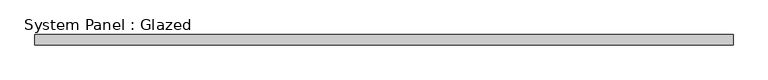
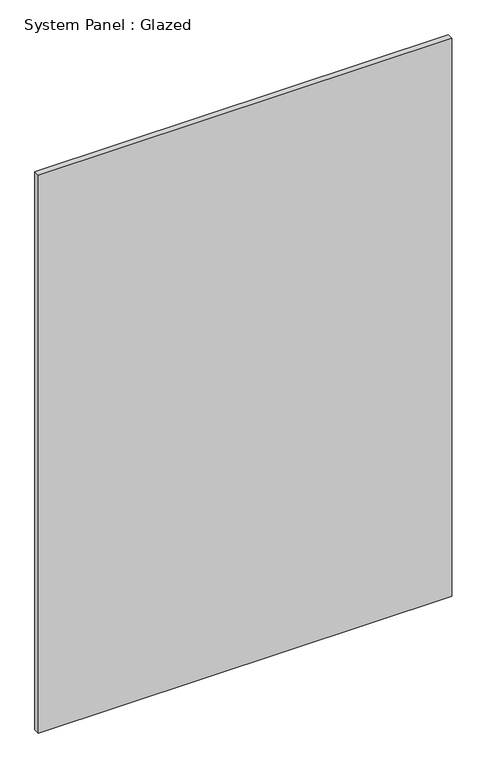
"""IFC4 building model written with IfcOpenShell, lengths in millimetres: plate geometry, System Panel : Glazed."""

from ifc_helpers import new_model, si_unit, origin, origin_with_axes, place, context, project, spatial, polyline, outline, extrude, source, transform, mapped, element, save


def system_panel_glazed_5990fd4e(model_context):
    return source(origin(), model_context, "Body", "SweptSolid", [
        extrude(outline(polyline([(832.5, 24.5), (-832.5, 24.5), (-832.5, 49.5), (832.5, 49.5), (832.5, 24.5)])), origin_with_axes(), (0.0, 0.0, 1.0), 2375.0),
    ])


if __name__ == "__main__":
    model = new_model("IFC4")
    model_context = context("Model", 3, world=origin())
    ifc_project = project(units=[si_unit("LENGTHUNIT", "METRE", prefix="MILLI")], contexts=[model_context])
    site = spatial("IfcSite", under=ifc_project)
    building = spatial("IfcBuilding", under=site)
    placement = place(None, origin())
    system_panel_glazed_shape = system_panel_glazed_5990fd4e(model_context)
    element("IfcPlate", 1, ObjectType="System Panel : Glazed", at=placement, inside=building, context=model_context, shape_type="MappedRepresentation", body=[
        mapped(system_panel_glazed_shape, transform((0.0, 0.0, 0.0), x_axis=(1.0, 0.0, 0.0), y_axis=(0.0, 1.0, 0.0), z_axis=(0.0, 0.0, 1.0))),
    ])
    save(model, "model.ifc")

# Revit data of these elements
# Element 1 (IfcPlate, "System Panel : Glazed")
#   Materials on its faces: "Glass"
# Materials
#   "Glass": class "Glass", colour RGB 218 227 224, transparency 0.85, Description = "Soda Lime Glass", Cost = 0
